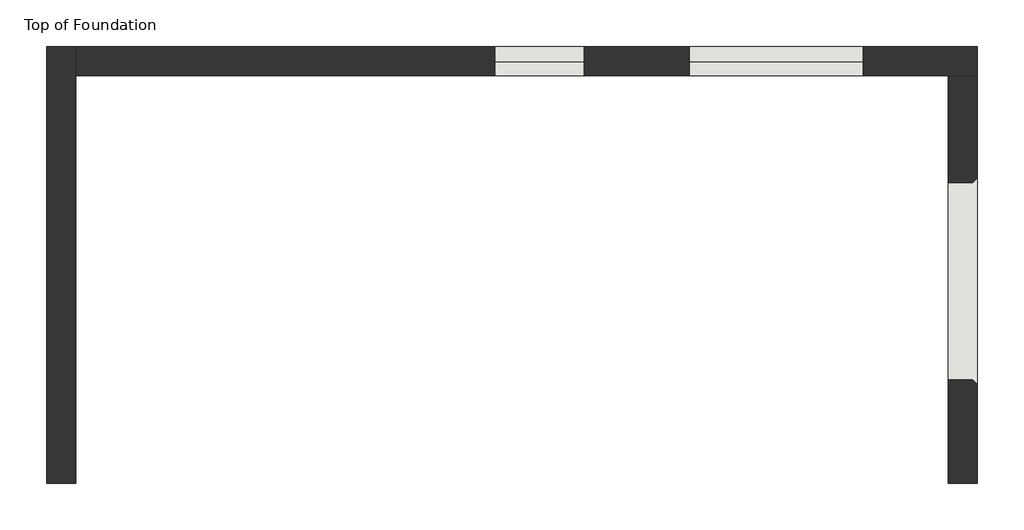
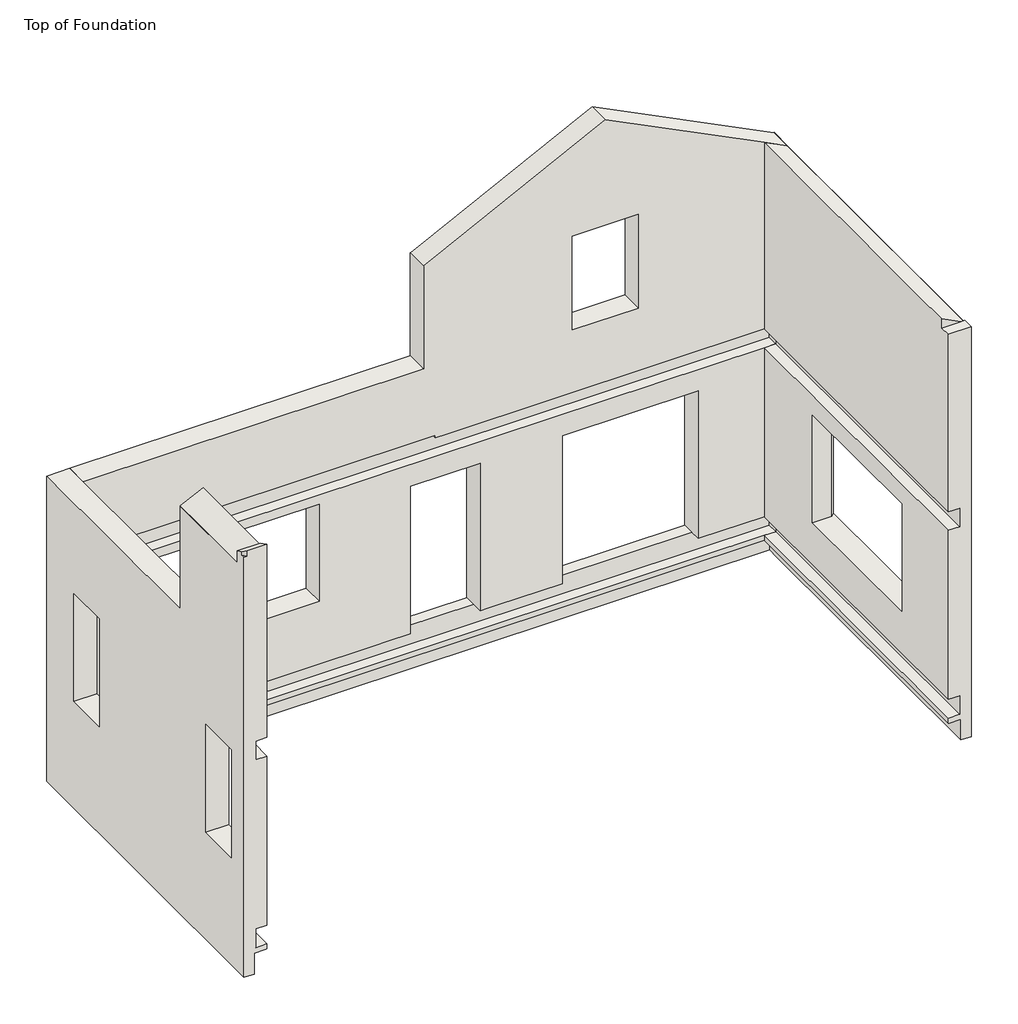
# One storey: 3 walls.
"""IFC4 building model written with IfcOpenShell, lengths in millimetres."""

from ifc_helpers import new_model, si_unit, origin, place, context, project, spatial, faceted_brep, element, save

model = new_model("IFC4")

# Units and contexts
model_context = context("Model", 3, world=origin())
ifc_project = project(units=[si_unit("LENGTHUNIT", "METRE", prefix="MILLI")], contexts=[model_context])

# Site, building, storey
site = spatial("IfcSite", under=ifc_project)
building = spatial("IfcBuilding", under=site)
storey = spatial("IfcBuildingStorey", under=building, Name="Top of Foundation", Elevation=-349.25)

# Walls
placement = place(None, origin())
element("IfcWall", 1, ObjectType="Exterior - Brick on Mtl. Stud", at=placement, inside=storey, context=model_context, shape_type="Brep", body=[
    faceted_brep([(-5671.6803068, 3152.0888758, -349.25), (-5671.6803068, 7558.9888758, -349.25), (-5671.6803068, 7876.4888758, -349.25), (-5671.6803068, 7876.4888758, 3810.0), (-5671.6803068, 7558.9888758, 3810.0), (-5671.6803068, 4676.0888758, 3810.0), (-5671.6803068, 4676.0888758, 5468.9375), (-5671.6803068, 4358.5888758, 5468.9375), (-5671.6803068, 3304.4888758, 5468.9375), (-5671.6803068, 3304.4888758, 5488.5342644), (-5671.6803068, 3152.0888758, 5564.7342644), (-5671.6803068, 3152.0888758, 2743.2), (-5671.6803068, 4358.5888758, 2743.2), (-5671.6803068, 4514.1638758, 2743.2), (-5671.6803068, 4514.1638758, 2781.3), (-5671.6803068, 4676.0888758, 2781.3), (-5671.6803068, 7558.9888758, 2781.3), (-5671.6803068, 7714.5638758, 2781.3), (-5671.6803068, 7714.5638758, 2470.15), (-5671.6803068, 7558.9888758, 2470.15), (-5671.6803068, 7219.2638758, 2470.15), (-5671.6803068, 7219.2638758, 914.4), (-5671.6803068, 6609.6638758, 914.4), (-5671.6803068, 6609.6638758, 2470.15), (-5671.6803068, 4066.4888758, 2470.15), (-5671.6803068, 4066.4888758, 914.4), (-5671.6803068, 3456.8888758, 914.4), (-5671.6803068, 3456.8888758, 2470.15), (-5671.6803068, 3152.0888758, 2470.15), (-5671.6803068, 3152.0888758, 0.0), (-5671.6803068, 7558.9888758, 0.0), (-5671.6803068, 7714.5638758, 0.0), (-5671.6803068, 7714.5638758, -273.05), (-5671.6803068, 7558.9888758, -273.05), (-5671.6803068, 3152.0888758, -273.05), (-5989.1803068, 3152.0888758, -654.05), (-5989.1803068, 3152.0888758, 5486.4), (-5989.1803068, 3199.7138758, 5486.4), (-5989.1803068, 3199.7138758, 5540.9217644), (-5989.1803068, 3304.4888758, 5488.5342644), (-5989.1803068, 3304.4888758, 5312.3217644), (-5989.1803068, 4676.0888758, 5312.3217644), (-5989.1803068, 4676.0888758, 3810.0), (-5989.1803068, 7876.4888758, 3810.0), (-5989.1803068, 7876.4888758, -654.05), (-5989.1803068, 3456.8888758, 2489.2), (-5989.1803068, 3456.8888758, 914.4), (-5989.1803068, 4066.4888758, 914.4), (-5989.1803068, 4066.4888758, 2489.2), (-5989.1803068, 6609.6638758, 2489.2), (-5989.1803068, 6609.6638758, 914.4), (-5989.1803068, 7219.2638758, 914.4), (-5989.1803068, 7219.2638758, 2489.2), (-5846.3053068, 7876.4888758, -349.25), (-5846.3053068, 7876.4888758, -654.05), (-5846.3053068, 3152.0888758, -654.05), (-5846.3053068, 3152.0888758, -349.25), (-5684.3803068, 3152.0888758, -349.25), (-5827.2553068, 3152.0888758, -273.05), (-5827.2553068, 3152.0888758, 0.0), (-5827.2553068, 3152.0888758, 2470.15), (-5827.2553068, 3152.0888758, 2743.2), (-5941.5553068, 3152.0888758, 5564.7342644), (-5941.5553068, 3152.0888758, 5486.4), (-5984.911778, 4676.0888758, 5312.3217644), (-5937.286778, 3304.4888758, 5336.1342644), (-5984.911778, 3304.4888758, 5312.3217644), (-5846.3053068, 7733.6138758, -349.25), (-5846.3053068, 7733.6138758, -654.05), (-5827.2553068, 3456.8888758, 2489.2), (-5827.2553068, 3456.8888758, 2470.15), (-5827.2553068, 4066.4888758, 2470.15), (-5827.2553068, 4066.4888758, 2489.2), (-5827.2553068, 6609.6638758, 2489.2), (-5827.2553068, 6609.6638758, 2470.15), (-5827.2553068, 7219.2638758, 2470.15), (-5827.2553068, 7219.2638758, 2489.2), (-5827.2553068, 7714.5638758, -273.05), (-5827.2553068, 7714.5638758, 0.0), (-5827.2553068, 7714.5638758, 2470.15), (-5827.2553068, 4514.1638758, 2470.15), (-5827.2553068, 4514.1638758, 2743.2), (-5827.2553068, 7714.5638758, 2781.3), (-5827.2553068, 4514.1638758, 2781.3)], [[[0, 1, 2, 3, 4, 5, 6, 7, 8, 9, 10, 11, 12, 13, 14, 15, 16, 17, 18, 19, 20, 21, 22, 23, 24, 25, 26, 27, 28, 29, 30, 31, 32, 33, 34]], [[35, 36, 37, 38, 39, 40, 41, 42, 43, 44], [45, 46, 47, 48], [49, 50, 51, 52]], [[3, 2, 53, 54, 44, 43]], [[36, 35, 55, 56, 57, 0, 34, 58, 59, 29, 28, 60, 61, 11, 10, 62, 63]], [[5, 4, 3, 43, 42]], [[6, 5, 42, 41, 64]], [[40, 39, 9, 8, 65, 66]], [[37, 36, 63]], [[37, 63, 62, 38]], [[8, 7, 6, 64, 66, 65]], [[41, 40, 66, 64]], [[10, 9, 39, 38, 62]], [[2, 1, 0, 57, 56, 67, 53]], [[53, 67, 56, 55, 68, 54]], [[55, 35, 44, 54, 68]], [[46, 45, 69, 70, 27, 26]], [[47, 46, 26, 25]], [[48, 47, 25, 24, 71, 72]], [[45, 48, 72, 69]], [[50, 49, 73, 74, 23, 22]], [[51, 50, 22, 21]], [[52, 51, 21, 20, 75, 76]], [[49, 52, 76, 73]], [[77, 58, 34, 33, 32]], [[78, 31, 30, 29, 59]], [[78, 77, 32, 31]], [[77, 78, 59, 58]], [[79, 75, 20, 19, 18]], [[71, 24, 23, 74, 80]], [[70, 60, 28, 27]], [[61, 81, 13, 12, 11]], [[60, 70, 69, 72, 71, 80, 74, 73, 76, 75, 79, 82, 83, 81, 61]], [[83, 82, 17, 16, 15, 14]], [[82, 79, 18, 17]], [[81, 83, 14, 13]]]),
])
element("IfcWall", 2, ObjectType="Exterior - Brick on Mtl. Stud", at=placement, inside=storey, context=model_context, shape_type="Brep", body=[
    faceted_brep([(-5671.6803068, 7558.9888758, -349.25), (3751.7196932, 7558.9888758, -349.25), (4069.2196932, 7558.9888758, -349.25), (4069.2196932, 7558.9888758, 5312.3217644), (4064.9511643, 7558.9888758, 5312.3217644), (3751.7196932, 7558.9888758, 5468.9375), (1554.6196932, 7558.9888758, 6567.4875), (-642.4803068, 7558.9888758, 5468.9375), (-955.711778, 7558.9888758, 5312.3217644), (-959.9803068, 7558.9888758, 5312.3217644), (-959.9803068, 7558.9888758, 3810.0), (-5671.6803068, 7558.9888758, 3810.0), (-5671.6803068, 7558.9888758, 2781.3), (-798.0553068, 7558.9888758, 2781.3), (-798.0553068, 7558.9888758, 2743.2), (-642.4803068, 7558.9888758, 2743.2), (3751.7196932, 7558.9888758, 2743.2), (3907.2946932, 7558.9888758, 2743.2), (3907.2946932, 7558.9888758, 2470.15), (3751.7196932, 7558.9888758, 2470.15), (43.3196932, 7558.9888758, 2470.15), (-77.3303068, 7558.9888758, 2470.15), (-1480.6803068, 7558.9888758, 2470.15), (-1601.3303068, 7558.9888758, 2470.15), (-5671.6803068, 7558.9888758, 2470.15), (-5671.6803068, 7558.9888758, 0.0), (-1601.3303068, 7558.9888758, 0.0), (-1480.6803068, 7558.9888758, 0.0), (-1144.1303068, 7558.9888758, 0.0), (-1144.1303068, 7558.9888758, 2159.0), (-178.9303068, 7558.9888758, 2159.0), (-178.9303068, 7558.9888758, 0.0), (-77.3303068, 7558.9888758, 0.0), (43.3196932, 7558.9888758, 0.0), (957.7196932, 7558.9888758, 0.0), (957.7196932, 7558.9888758, 2159.0), (2837.3196932, 7558.9888758, 2159.0), (2837.3196932, 7558.9888758, 0.0), (3751.7196932, 7558.9888758, 0.0), (3907.2946932, 7558.9888758, 0.0), (3907.2946932, 7558.9888758, -273.05), (3751.7196932, 7558.9888758, -273.05), (-5671.6803068, 7558.9888758, -273.05), (1097.4196932, 7558.9888758, 3657.6), (1097.4196932, 7558.9888758, 5029.2), (2011.8196932, 7558.9888758, 5029.2), (2011.8196932, 7558.9888758, 3657.6), (-2399.8428068, 7558.9888758, 2336.8), (-2399.8428068, 7558.9888758, 914.4), (-4838.2428068, 7558.9888758, 914.4), (-4838.2428068, 7558.9888758, 2336.8), (4069.2196932, 7876.4888758, 5312.3217644), (4069.2196932, 7876.4888758, -654.05), (-4007.9803068, 7876.4888758, -654.05), (-4312.7803068, 7876.4888758, -654.05), (-5846.3053068, 7876.4888758, -654.05), (-5846.3053068, 7876.4888758, -349.25), (-5671.6803068, 7876.4888758, -349.25), (-5671.6803068, 7876.4888758, 3810.0), (-959.9803068, 7876.4888758, 3810.0), (-959.9803068, 7876.4888758, 5312.3217644), (-955.711778, 7876.4888758, 5312.3217644), (1554.6196932, 7876.4888758, 6567.4875), (4064.9511643, 7876.4888758, 5312.3217644), (1097.4196932, 7876.4888758, 5029.2), (1097.4196932, 7876.4888758, 3657.6), (2011.8196932, 7876.4888758, 3657.6), (2011.8196932, 7876.4888758, 5029.2), (-1144.1303068, 7876.4888758, 2159.0), (-1144.1303068, 7876.4888758, 0.0), (-178.9303068, 7876.4888758, 0.0), (-178.9303068, 7876.4888758, 2159.0), (-2399.8428068, 7876.4888758, 914.4), (-2399.8428068, 7876.4888758, 2336.8), (-4838.2428068, 7876.4888758, 2336.8), (-4838.2428068, 7876.4888758, 914.4), (2837.3196932, 7876.4888758, 0.0), (2837.3196932, 7876.4888758, 2159.0), (957.7196932, 7876.4888758, 2159.0), (957.7196932, 7876.4888758, 0.0), (-5671.6803068, 7733.6138758, -349.25), (-5671.6803068, 7714.5638758, -273.05), (-5671.6803068, 7714.5638758, 0.0), (-5671.6803068, 7714.5638758, 2470.15), (-5671.6803068, 7714.5638758, 2781.3), (4069.2196932, 7733.6138758, -349.25), (4069.2196932, 7733.6138758, -654.05), (-4312.7803068, 7733.6138758, -349.25), (-4007.9803068, 7733.6138758, -349.25), (3926.3446932, 7733.6138758, -349.25), (-5846.3053068, 7733.6138758, -349.25), (-5846.3053068, 7733.6138758, -654.05), (-4312.7803068, 7733.6138758, -654.05), (-4007.9803068, 7733.6138758, -654.05), (3926.3446932, 7733.6138758, -654.05), (-1144.1303068, 7714.5638758, 0.0), (-178.9303068, 7714.5638758, 0.0), (2837.3196932, 7714.5638758, 0.0), (957.7196932, 7714.5638758, 0.0), (3907.2946932, 7714.5638758, -273.05), (3907.2946932, 7714.5638758, 0.0), (3907.2946932, 7714.5638758, 2470.15), (-798.0553068, 7714.5638758, 2470.15), (-798.0553068, 7714.5638758, 2743.2), (3907.2946932, 7714.5638758, 2743.2), (-798.0553068, 7714.5638758, 2781.3)], [[[0, 1, 2, 3, 4, 5, 6, 7, 8, 9, 10, 11, 12, 13, 14, 15, 16, 17, 18, 19, 20, 21, 22, 23, 24, 25, 26, 27, 28, 29, 30, 31, 32, 33, 34, 35, 36, 37, 38, 39, 40, 41, 42], [43, 44, 45, 46], [47, 48, 49, 50]], [[51, 52, 53, 54, 55, 56, 57, 58, 59, 60, 61, 62, 63], [64, 65, 66, 67], [68, 69, 70, 71], [72, 73, 74, 75], [76, 77, 78, 79]], [[11, 58, 57, 80, 0, 42, 81, 82, 25, 24, 83, 84, 12]], [[3, 2, 85, 86, 52, 51]], [[11, 10, 59, 58]], [[10, 9, 60, 59]], [[60, 9, 8, 61]], [[8, 7, 6, 62, 61]], [[6, 5, 4, 63, 62]], [[3, 51, 63, 4]], [[2, 1, 0, 80, 87, 88, 89, 85]], [[85, 89, 88, 87, 80, 90, 91, 92, 93, 94, 86]], [[52, 86, 94, 93, 92, 91, 55, 54, 53]], [[90, 80, 57, 56]], [[55, 91, 90, 56]], [[65, 64, 44, 43]], [[66, 65, 43, 46]], [[67, 66, 46, 45]], [[64, 67, 45, 44]], [[29, 28, 95, 69, 68]], [[30, 29, 68, 71]], [[31, 30, 71, 70, 96]], [[70, 69, 95, 96]], [[48, 72, 75, 49]], [[73, 47, 50, 74]], [[72, 48, 47, 73]], [[74, 50, 49, 75]], [[77, 76, 97, 37, 36]], [[78, 77, 36, 35]], [[79, 78, 35, 34, 98]], [[76, 79, 98, 97]], [[40, 99, 81, 42, 41]], [[97, 100, 39, 38, 37]], [[96, 98, 34, 33, 32, 31]], [[82, 95, 28, 27, 26, 25]], [[99, 100, 97, 98, 96, 95, 82, 81]], [[100, 99, 40, 39]], [[83, 24, 23, 22, 21, 20, 19, 18, 101, 102]], [[103, 104, 17, 16, 15, 14]], [[83, 102, 101, 104, 103, 105, 84]], [[104, 101, 18, 17]], [[84, 105, 13, 12]], [[105, 103, 14, 13]]]),
])
element("IfcWall", 3, ObjectType="Exterior - Brick on Mtl. Stud", at=placement, inside=storey, context=model_context, shape_type="Brep", body=[
    faceted_brep([(3751.7196932, 7558.9888758, -349.25), (3751.7196932, 3152.0888758, -349.25), (3751.7196932, 3152.0888758, -273.05), (3751.7196932, 7558.9888758, -273.05), (3751.7196932, 3304.4888758, 5336.1342644), (3751.7196932, 3304.4888758, 5468.9375), (3751.7196932, 3844.2388758, 5468.9375), (3751.7196932, 3964.8888758, 5468.9375), (3751.7196932, 7558.9888758, 5468.9375), (3751.7196932, 7558.9888758, 2743.2), (3751.7196932, 3964.8888758, 2743.2), (3751.7196932, 3844.2388758, 2743.2), (3751.7196932, 3152.0888758, 2743.2), (3751.7196932, 3152.0888758, 5336.1342644), (3751.7196932, 7558.9888758, 0.0), (3751.7196932, 3152.0888758, 0.0), (3751.7196932, 3152.0888758, 2470.15), (3751.7196932, 7558.9888758, 2470.15), (3751.7196932, 6404.8763758, 2184.4), (3751.7196932, 4271.2763758, 2184.4), (3751.7196932, 4271.2763758, 609.6), (3751.7196932, 6404.8763758, 609.6), (4069.2196932, 3152.0888758, 5336.1342644), (4069.2196932, 3152.0888758, -654.05), (4069.2196932, 7571.6888758, -654.05), (4069.2196932, 7733.6138758, -654.05), (4069.2196932, 7733.6138758, -349.25), (4069.2196932, 7558.9888758, -349.25), (4069.2196932, 7558.9888758, 5312.3217644), (4069.2196932, 3304.4888758, 5312.3217644), (4069.2196932, 3304.4888758, 5336.1342644), (4069.2196932, 4221.8849671, 2184.4), (4069.2196932, 6454.2677845, 2184.4), (4069.2196932, 6454.2677845, 609.6), (4069.2196932, 4221.8849671, 609.6), (3907.2946932, 3152.0888758, 2743.2), (3907.2946932, 3152.0888758, 2470.15), (3907.2946932, 3152.0888758, 0.0), (3907.2946932, 3152.0888758, -273.05), (3764.4196932, 3152.0888758, -349.25), (3926.3446932, 3152.0888758, -349.25), (3926.3446932, 3152.0888758, -654.05), (4064.9511643, 7558.9888758, 5312.3217644), (3926.3446932, 7558.9888758, -349.25), (3907.2946932, 7558.9888758, -273.05), (3907.2946932, 7558.9888758, 0.0), (3907.2946932, 7558.9888758, 2470.15), (3907.2946932, 7558.9888758, 2743.2), (4064.9511643, 3304.4888758, 5312.3217644), (4017.3261643, 3304.4888758, 5336.1342644), (3926.3446932, 7571.6888758, -349.25), (3926.3446932, 7733.6138758, -349.25), (3926.3446932, 7733.6138758, -654.05), (3926.3446932, 7571.6888758, -654.05), (4019.8282845, 6404.8763758, 2184.4), (4019.8282845, 4271.2763758, 2184.4), (4019.8282845, 6404.8763758, 609.6), (4019.8282845, 4271.2763758, 609.6)], [[[0, 1, 2, 3]], [[4, 5, 6, 7, 8, 9, 10, 11, 12, 13]], [[14, 15, 16, 17], [18, 19, 20, 21]], [[22, 23, 24, 25, 26, 27, 28, 29, 30], [31, 32, 33, 34]], [[23, 22, 13, 12, 35, 36, 16, 15, 37, 38, 2, 1, 39, 40, 41]], [[42, 28, 27, 43, 0, 3, 44, 45, 14, 17, 46, 47, 9, 8]], [[30, 29, 48, 49]], [[4, 13, 22, 30, 49]], [[8, 7, 6, 5, 49, 48, 42]], [[29, 28, 42, 48]], [[5, 4, 49]], [[1, 0, 43, 40, 39]], [[40, 43, 50, 51, 52, 53, 41]], [[23, 41, 53, 52, 25, 24]], [[51, 50, 43, 27, 26]], [[25, 52, 51, 26]], [[54, 32, 31, 55, 19, 18]], [[56, 21, 20, 57, 34, 33]], [[54, 18, 21, 56]], [[19, 55, 57, 20]], [[55, 31, 34, 57]], [[32, 54, 56, 33]], [[38, 44, 3, 2]], [[45, 37, 15, 14]], [[44, 38, 37, 45]], [[36, 46, 17, 16]], [[47, 35, 12, 11, 10, 9]], [[46, 36, 35, 47]]]),
])

save(model, "model.ifc")

# Revit data of these elements
# Type "Exterior - Brick on Mtl. Stud"
#   Assembly Code = "B2010158"
#   Layers, outside or top first: 0' - 3 5/8" "Brick, Common" (function 4); 0' - 2" "Air" (function 3); 0' - 0" "Air Infiltration Barrier" (function 100); 0' - 0 3/4" "Plywood, Sheathing" (function 2); 0' - 5 1/2" "Metal Stud Layer" (function 1); 0' - 0" "Vapor Retarder" (function 100); 0' - 0 5/8" "Gypsum Wall Board" (function 5)
# Elements 1, 2 (IfcWall, "Exterior - Brick on Mtl. Stud")
#   built-in parameter 1012829 = -1 (stored number, unit not read)
#   Top Offset = 0' - 0"
#   Base Offset = 0' - 0"
#   wall height = 19' - 1 3/4"
#   Phase Created = New Construction
#   Base Constraint = Top of Foundation
#   Top Constraint = Roof
#   Materials on its faces: "Default Wall", "Brick, Common", "Gypsum Wall Board"
# Element 3 (IfcWall, "Exterior - Brick on Mtl. Stud")
#   built-in parameter 1012829 = -1 (stored number, unit not read)
#   Top Offset = 0' - 0"
#   Base Offset = 0' - 0"
#   wall height = 19' - 1 3/4"
#   Phase Created = New Construction
#   Base Constraint = Top of Foundation
#   Top Constraint = Roof
#   Materials on its faces: "Default Wall", "Gypsum Wall Board", "Brick, Common"
# Materials
#   "Brick, Common": class "Masonry", colour RGB 170 98 104, transparency 0, Keynote = "04 21 00.A1", Description = "Common brick", Cost = 0
#   "Air": class "Gas", colour RGB 255 255 255, transparency 0, Description = "Air", Cost = 0
#   "Air Infiltration Barrier": class "Generic", colour RGB 127 127 127, transparency 0, Description = "physical material", Cost = 0
#   "Plywood, Sheathing": class "Wood", colour RGB 193 140 64, transparency 0, Description = "Plywood, sheathing grade", Cost = 0
#   "Metal Stud Layer": class "Metal", colour RGB 199 199 199, transparency 0, Description = "Light gauge steel framing, thermal air layer", Cost = 0
#   "Vapor Retarder": class "Generic", colour RGB 127 127 127, transparency 0, Description = "Polyethylene film membrane", Cost = 0
#   "Gypsum Wall Board": class "Generic", colour RGB 127 127 127, transparency 0, Description = "Gypsum Wall Board", Cost = 0
#   "Default Wall": class "Miscellaneous", colour RGB 128 128 128, transparency 0, Cost = 0
